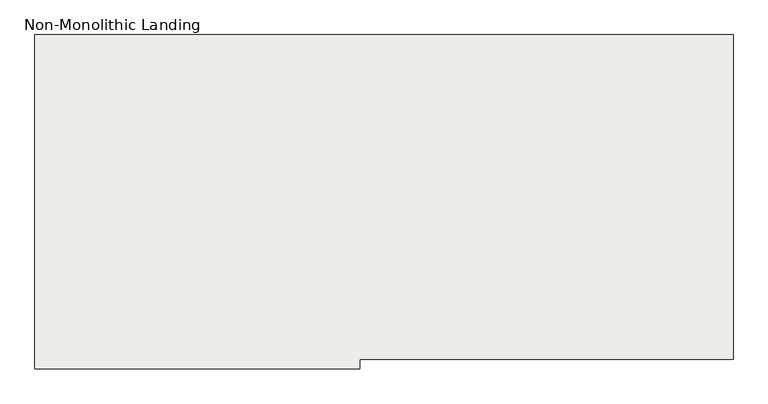
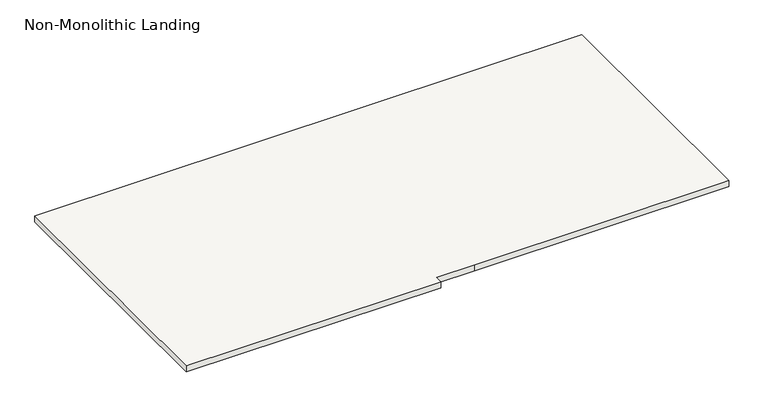
"""IFC4 building model written with IfcOpenShell, lengths in millimetres: slab geometry, Non-Monolithic Landing."""

from ifc_helpers import new_model, si_unit, frame, origin, place, context, project, spatial, polyline, outline, extrude, source, transform, mapped, element, save


def non_monolithic_landing_5ffb325b(model_context):
    return source(origin(), model_context, "Body", "SweptSolid", [
        extrude(outline(polyline([(12700.0002443, 23469.9999999), (12700.0002443, 25529.9999999), (17000.0002442, 25529.9999999), (17000.0002442, 23529.9999999), (15000.0002442, 23529.9999999), (14700.0002443, 23529.9999999), (14700.0002443, 23469.9999999), (12700.0002443, 23469.9999999)])), frame((0.0, 0.0, 22283.3333333), z_axis=(0.0, 0.0, 1.0), x_axis=(1.0, 0.0, 0.0)), (0.0, 0.0, 1.0), 50.0),
    ])


if __name__ == "__main__":
    model = new_model("IFC4")
    model_context = context("Model", 3, world=origin())
    ifc_project = project(units=[si_unit("LENGTHUNIT", "METRE", prefix="MILLI")], contexts=[model_context])
    site = spatial("IfcSite", under=ifc_project)
    building = spatial("IfcBuilding", under=site)
    placement = place(None, origin())
    non_monolithic_landing_shape = non_monolithic_landing_5ffb325b(model_context)
    element("IfcSlab", 1, ObjectType="Non-Monolithic Landing", at=placement, inside=building, context=model_context, shape_type="MappedRepresentation", body=[
        mapped(non_monolithic_landing_shape, transform((0.0, 0.0, 0.0), x_axis=(1.0, 0.0, 0.0), y_axis=(0.0, 1.0, 0.0), z_axis=(0.0, 0.0, 1.0))),
    ])
    save(model, "model.ifc")
